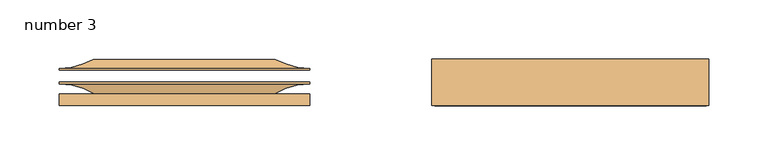
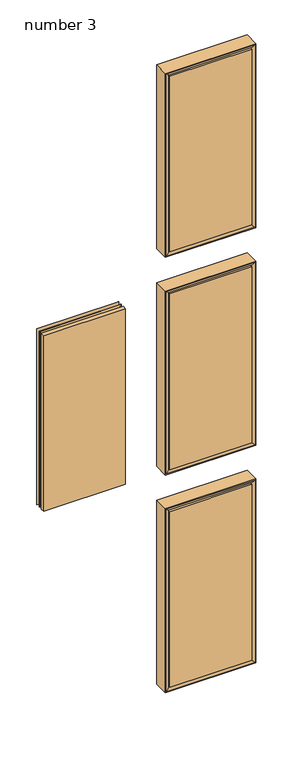
# IFC4 building model written with IfcOpenShell, lengths in millimetres: door geometry, Door-Interior-Karona-K5660-6_Panel : number 3.
# Revit data of these elements (continued)
# Type "Door-Interior-Karona-K5660-6_Panel : number 3" (continued)
#   Daylight Opening Height = 0' - 0"
#   Bottom Rail Height = 0' - 8 1/2"
#   3D Open Angle = 0.00°
#   Thickness = 0' - 1 3/4"
#   Stop Thickness = 0' - 0 1/2"
#   Stop Depth = 0' - 1 3/8"
#   Rough Width = 2' - 9 29/32"
#   Rough Height = 6' - 8 61/64"
#   Rabbet Width = 0' - 1 3/4"
#   Jamb Offset = 0' - 0 61/64"
#   Hinge Offset = 0' - 0 3/4"
#   Jamb Thickness = 0' - 0 29/32"
#   Ext. Frame Thickness = 0' - 0 5/8"
#   Int. Frame Thickness = 0' - 0 5/8"
#   Height = 6' - 8"
#   Width = 2' - 8"
#   3D Angle = 0.00°
#   Trim Visible = yes
#   Square Sticking Profile = no
#   Raised Panel Door = yes
#   Ovolo Sticking Profile = yes
#   Ogee Sticking Profile = no
#   Mission Sticking Profile = no
#   Hinge Visible = yes
#   Glass Panel Door = no
#   Flat Panel Door = no
#   Edition number = 1
#   Define Thermal Properties by = 1
#   Trim Material = Wood - Karona - Red Oak
#   Top Rail Material = Wood - Karona - Red Oak
#   Stile Material = Wood - Karona - Red Oak
#   Sticking Material = Wood - Karona - Red Oak
#   Jamb Material = Wood - Karona - Red Oak
#   Interior Panel = Wood - Karona - Red Oak
#   Door Panel Material = Wood - Karona - Red Oak
#   Bottom Rail Material = Wood - Karona - Red Oak
#   Visual Light Transmittance = 0
#   Solar Heat Gain Coefficient = 0
#   Construction Type = (empty or 0)
#   Function = (empty or 0)
#   Wall Closure = (empty or 0)
# Element 1 (IfcDoor, "Door-Interior-Karona-K5660-6_Panel : number 3")
#   Materials on its faces: "Wood - Karona - Red Oak"
# Materials
#   "Wood - Karona - Red Oak": class "Wood", colour RGB 153 121 89, transparency 0, Description = "Quercus Rubra", Cost = 0
